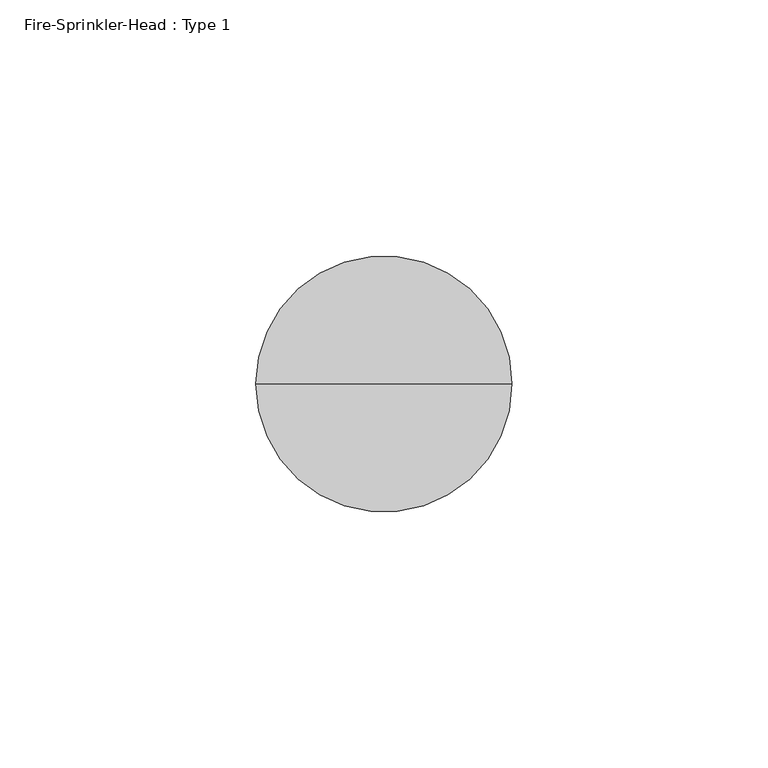
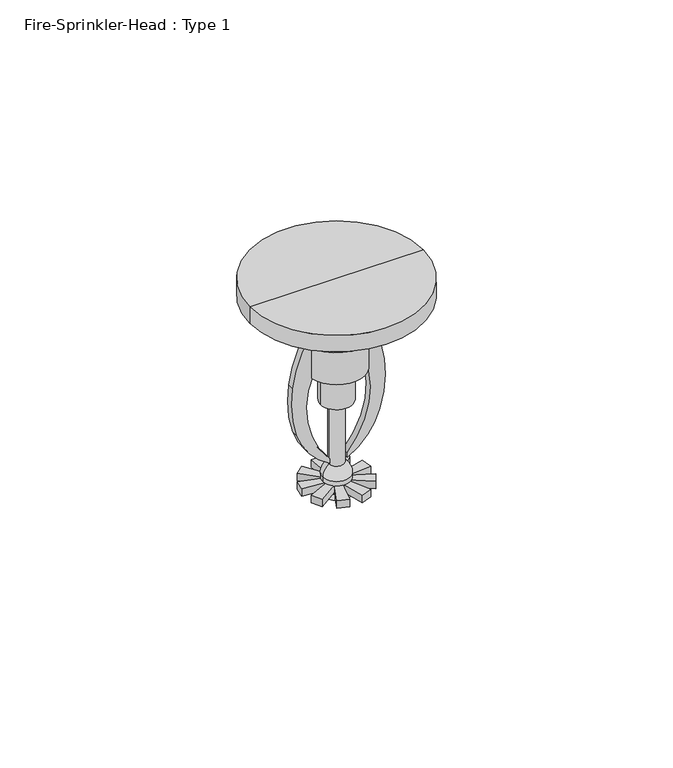
"""IFC4 building model written with IfcOpenShell, lengths in millimetres: alarm geometry, Fire-Sprinkler-Head : Type 1."""

import ifcopenshell
import ifcopenshell.guid

model = None  # the IFC model being written
_history = None  # IfcOwnerHistory: only IFC2X3 demands one
_inside = {}  # id of a spatial element -> (the spatial element, [elements in it])
_under = {}  # id of a project, library or spatial element -> (it, [spatial elements below it])
_declared = {}  # id of a project -> (the project, [libraries it declares])
_typed = {}  # id of a type object -> (the type object, [elements of that type])
_made_of = {}  # id of a material, layer set ... -> (it, [elements and type objects made of it])


def new_model(schema):
    """Start an empty IFC model of exactly this schema.

    Asked for "IFC4X3", IfcOpenShell would pick the latest addendum, in which some entities
    have other attributes; the version numbers below select the first issue.
    IFC2X3 requires an IfcOwnerHistory on every rooted entity: one is made here for all.
    """
    global model, _history
    if schema == "IFC4X3":
        model = ifcopenshell.file(schema_version=(4, 3, 0, 0))
    else:
        model = ifcopenshell.file(schema=schema)
    _inside.clear()
    _under.clear()
    _declared.clear()
    _typed.clear()
    _made_of.clear()
    _history = None
    if model.schema == "IFC2X3":
        org = make("IfcOrganization", Name="unknown")
        user = make(
            "IfcPersonAndOrganization",
            ThePerson=make("IfcPerson", FamilyName="unknown"),
            TheOrganization=org,
        )
        app = make(
            "IfcApplication",
            ApplicationDeveloper=org,
            Version="unknown",
            ApplicationFullName="unknown",
            ApplicationIdentifier="unknown",
        )
        _history = make(
            "IfcOwnerHistory",
            OwningUser=user,
            OwningApplication=app,
            ChangeAction="ADDED",
            CreationDate=0,
        )
    return model


def make(cls, **values):
    """One entity of the class cls with the attributes given. An attribute that is None is left unset."""
    return model.create_entity(
        cls, **{name: value for name, value in values.items() if value is not None}
    )


def rooted(cls, **values):
    """An entity with a GlobalId (a new one), such as an element, a storey or a relation."""
    return make(cls, GlobalId=ifcopenshell.guid.new(), OwnerHistory=_history, **values)


def si_unit(unit_type, name, prefix=None):
    """IfcSIUnit, for example si_unit("LENGTHUNIT", "METRE", prefix="MILLI")."""
    return make("IfcSIUnit", UnitType=unit_type, Prefix=prefix, Name=name)


def assignment(units):
    """IfcUnitAssignment: the units of a project."""
    return None if units is None else make("IfcUnitAssignment", Units=units)


def point(xyz):
    """IfcCartesianPoint."""
    return None if xyz is None else make("IfcCartesianPoint", Coordinates=xyz)


def direction(xyz):
    """IfcDirection."""
    return None if xyz is None else make("IfcDirection", DirectionRatios=xyz)


def frame(location, z_axis=None, x_axis=None):
    """IfcAxis2Placement3D, a coordinate frame: its origin and axes. An axis left out is left unset."""
    return make(
        "IfcAxis2Placement3D",
        Location=point(location),
        Axis=direction(z_axis),
        RefDirection=direction(x_axis),
    )


def frame_2d(location, x_axis=None):
    """IfcAxis2Placement2D, a coordinate frame in the plane: its origin and x axis."""
    return make(
        "IfcAxis2Placement2D", Location=point(location), RefDirection=direction(x_axis)
    )


def origin():
    """The frame at (0, 0, 0) with its axes left unset."""
    return frame((0.0, 0.0, 0.0))


def place(relative_to, where):
    """IfcLocalPlacement: puts the frame where relative to a parent placement (None: the world)."""
    return make(
        "IfcLocalPlacement", PlacementRelTo=relative_to, RelativePlacement=where
    )


def context(
    kind, dimensions, precision=None, world=None, true_north=None, identifier=None
):
    """IfcGeometricRepresentationContext, for example the 3D "Model" context."""
    return make(
        "IfcGeometricRepresentationContext",
        ContextIdentifier=identifier,
        ContextType=kind,
        CoordinateSpaceDimension=dimensions,
        Precision=precision,
        WorldCoordinateSystem=world,
        TrueNorth=true_north,
    )


def project(units=None, contexts=None):
    """IfcProject with its units and contexts."""
    return rooted(
        "IfcProject",
        Name="project",
        RepresentationContexts=contexts,
        UnitsInContext=assignment(units),
    )


def spatial(cls, under=None, at=None, **own):
    """A site, building, storey or space (cls), placed at a placement, below another one or the project."""
    s = rooted(cls, ObjectPlacement=at, **own)
    if under is not None:
        _under.setdefault(under.id(), (under, []))[1].append(s)
    return s


def polyline(points):
    """IfcPolyline through the points."""
    return make("IfcPolyline", Points=[point(p) for p in points])


def circle_curve(where, radius):
    """IfcCircle in the frame where."""
    return make("IfcCircle", Position=where, Radius=radius)


def ellipse_curve(where, semi_axis1, semi_axis2):
    """IfcEllipse in the frame where."""
    return make(
        "IfcEllipse", Position=where, SemiAxis1=semi_axis1, SemiAxis2=semi_axis2
    )


def trimmed(basis, trim1, trim2, sense, master):
    """IfcTrimmedCurve: the piece of a basis curve between two trims."""
    return make(
        "IfcTrimmedCurve",
        BasisCurve=basis,
        Trim1=trim1,
        Trim2=trim2,
        SenseAgreement=sense,
        MasterRepresentation=master,
    )


def segment(curve, same_sense, transition):
    """IfcCompositeCurveSegment."""
    return make(
        "IfcCompositeCurveSegment",
        Transition=transition,
        SameSense=same_sense,
        ParentCurve=curve,
    )


def composite_curve(segments, self_intersect=None):
    """IfcCompositeCurve: segments joined end to end."""
    return make("IfcCompositeCurve", Segments=segments, SelfIntersect=self_intersect)


def outline(outer, holes=None, kind="AREA"):
    """IfcArbitraryClosedProfileDef: a profile drawn as a closed curve; with holes, ...WithVoids."""
    if holes is None:
        return make("IfcArbitraryClosedProfileDef", ProfileType=kind, OuterCurve=outer)
    return make(
        "IfcArbitraryProfileDefWithVoids",
        ProfileType=kind,
        OuterCurve=outer,
        InnerCurves=holes,
    )


def extrude(swept, where, along, depth):
    """IfcExtrudedAreaSolid: the profile swept, set in the frame where, extruded along a direction by depth."""
    return make(
        "IfcExtrudedAreaSolid",
        SweptArea=swept,
        Position=where,
        ExtrudedDirection=direction(along),
        Depth=depth,
    )


def shape(context_of_items, identifier, shape_type, items):
    """IfcShapeRepresentation: the items that make up one representation, for example the "Body"."""
    return make(
        "IfcShapeRepresentation",
        ContextOfItems=context_of_items,
        RepresentationIdentifier=identifier,
        RepresentationType=shape_type,
        Items=items,
    )


def source(mapping_origin, context_of_items, identifier, shape_type, items):
    """IfcRepresentationMap: a shape defined once, which mapped items show again and again."""
    return make(
        "IfcRepresentationMap",
        MappingOrigin=mapping_origin,
        MappedRepresentation=shape(context_of_items, identifier, shape_type, items),
    )


def transform(
    local_origin,
    x_axis=None,
    y_axis=None,
    z_axis=None,
    scale=None,
    scale2=None,
    scale3=None,
    uniform=True,
):
    """IfcCartesianTransformationOperator3D, or its non-uniform kind. x_axis, y_axis, z_axis: its Axis1, 2, 3."""
    if uniform:
        return make(
            "IfcCartesianTransformationOperator3D",
            Axis1=direction(x_axis),
            Axis2=direction(y_axis),
            LocalOrigin=point(local_origin),
            Scale=scale,
            Axis3=direction(z_axis),
        )
    return make(
        "IfcCartesianTransformationOperator3DnonUniform",
        Axis1=direction(x_axis),
        Axis2=direction(y_axis),
        LocalOrigin=point(local_origin),
        Scale=scale,
        Axis3=direction(z_axis),
        Scale2=scale2,
        Scale3=scale3,
    )


def mapped(mapping_source, mapping_target):
    """IfcMappedItem: shows the shape of a source again, moved by a transform."""
    return make(
        "IfcMappedItem", MappingSource=mapping_source, MappingTarget=mapping_target
    )


def made_of(thing, what):
    """Note that an element or type object is made of a material, layer set ...; save() writes the relation."""
    if what is not None:
        _made_of.setdefault(what.id(), (what, []))[1].append(thing)
    return thing


def element(
    cls,
    number,
    at=None,
    inside=None,
    cuts=None,
    type_object=None,
    material=None,
    context=None,
    identifier="Body",
    shape_type=None,
    held_by="IfcProductDefinitionShape",
    body=None,
    shapes=None,
    **own,
):
    """One element of the class cls, such as IfcWall. Its Tag is "e" and its number.

    at: its placement. inside: the storey or other place that contains it. cuts: it is an
    opening in that element (IfcRelVoidsElement). A single representation is given by context,
    identifier, shape_type and body (its items); several are given by shapes. held_by: the class
    of the entity that holds the representations. save() writes the other relations.
    """
    e = rooted(cls, Tag="e%d" % number, ObjectPlacement=at, **own)
    if body is not None:
        shapes = [shape(context, identifier, shape_type, body)]
    if shapes is not None:
        e.Representation = make(held_by, Representations=shapes)
    if inside is not None:
        _inside.setdefault(inside.id(), (inside, []))[1].append(e)
    if cuts is not None:
        rooted(
            "IfcRelVoidsElement", RelatingBuildingElement=cuts, RelatedOpeningElement=e
        )
    if type_object is not None:
        _typed.setdefault(type_object.id(), (type_object, []))[1].append(e)
    return made_of(e, material)


def aggregate(whole, parts):
    """IfcRelAggregates: a whole, such as a stair, and the parts it consists of."""
    return rooted("IfcRelAggregates", RelatingObject=whole, RelatedObjects=parts)


def save(model, path):
    """Write the relations noted so far, then the file.

    IfcRelAggregates (storeys below a building ...), IfcRelContainedInSpatialStructure (elements
    in a storey), IfcRelDefinesByType, IfcRelAssociatesMaterial and IfcRelDeclares: one each for
    every whole, place, type object, material and project.
    """
    for whole, parts in _under.values():
        aggregate(whole, parts)
    for where, things in _inside.values():
        rooted(
            "IfcRelContainedInSpatialStructure",
            RelatedElements=things,
            RelatingStructure=where,
        )
    for kind, things in _typed.values():
        rooted("IfcRelDefinesByType", RelatedObjects=things, RelatingType=kind)
    for what, things in _made_of.values():
        rooted("IfcRelAssociatesMaterial", RelatedObjects=things, RelatingMaterial=what)
    for by, libraries in _declared.values():
        rooted("IfcRelDeclares", RelatingContext=by, RelatedDefinitions=libraries)
    model.write(path)


def plane_surface(at):
    """IfcPlane: the flat surface through the origin of the frame at, square to its z axis."""
    return make("IfcPlane", Position=at)


def cylinder_surface(at, radius):
    """IfcCylindricalSurface: all points at the distance radius from the z axis of the frame at."""
    return make("IfcCylindricalSurface", Position=at, Radius=radius)


def revolved_surface(curve, axis_point, axis_direction):
    """IfcSurfaceOfRevolution: the curve turned about the line through axis_point along axis_direction."""
    return make(
        "IfcSurfaceOfRevolution",
        SweptCurve=make("IfcArbitraryOpenProfileDef", ProfileType="CURVE", Curve=curve),
        AxisPosition=make("IfcAxis1Placement", Location=point(axis_point), Axis=direction(axis_direction)),
    )


def advanced_brep(points, edges, surfaces, faces):
    """IfcAdvancedBrep: a solid bounded by faces that lie on surfaces and meet in shared edges.

    An edge is (start, end): straight between two places in points (the first is 0);
    or (start, end, curve); or (start, end, curve, False) where it runs against its curve.
    A face is (place in surfaces, loops), or (place, loops, False) where it looks against
    its surface's normal. A loop lists edges by number (the first is 1), with a minus sign
    where the edge is run from its end to its start. The first loop is the outer one.
    """
    corners = [point(p) for p in points]
    vertices = [make("IfcVertexPoint", VertexGeometry=c) for c in corners]
    made = []
    for start, end, *more in edges:
        made.append(
            make(
                "IfcEdgeCurve",
                EdgeStart=vertices[start],
                EdgeEnd=vertices[end],
                EdgeGeometry=more[0] if more else make("IfcPolyline", Points=[corners[start], corners[end]]),
                SameSense=more[1] if len(more) > 1 else True,
            )
        )
    hull = []
    for where, loops, *sense in faces:
        bounds = []
        for j, loop in enumerate(loops):
            ring = [make("IfcOrientedEdge", EdgeElement=made[abs(k) - 1], Orientation=k > 0) for k in loop]
            bounds.append(
                make(
                    "IfcFaceOuterBound" if j == 0 else "IfcFaceBound",
                    Bound=make("IfcEdgeLoop", EdgeList=ring),
                    Orientation=True,
                )
            )
        hull.append(make("IfcAdvancedFace", Bounds=bounds, FaceSurface=surfaces[where], SameSense=sense[0] if sense else True))
    return make("IfcAdvancedBrep", Outer=make("IfcClosedShell", CfsFaces=hull))


def fire_sprinkler_head_type_1_89d12226(model_context):
    return source(origin(), model_context, "Body", "SolidModel", [
        extrude(outline(composite_curve([segment(polyline([(3978.349287, 0.0), (3978.349287, 4.8492465)]), True, "CONTINUOUS"), segment(trimmed(circle_curve(frame_2d((3963.8626562, -16.7101966)), 25.9744501), [point((3978.349287, 4.8492465))], [point((3946.4410747, 2.555331))], True, "CARTESIAN"), True, "CONTINUOUS"), segment(polyline([(3946.4410747, 2.555331), (3945.0501011, 2.555331)]), True, "CONTINUOUS"), segment(trimmed(circle_curve(frame_2d((3962.5874819, -7.1839127)), 20.0602242), [point((3945.0501011, 2.555331))], [point((3956.7072905, 11.9951369))], False, "CARTESIAN"), True, "CONTINUOUS"), segment(trimmed(circle_curve(frame_2d((3966.9398015, -21.3795994)), 34.9081266), [point((3956.7072905, 11.9951369))], [point((3971.4511948, 13.2357821))], False, "CARTESIAN"), True, "CONTINUOUS"), segment(trimmed(circle_curve(frame_2d((3966.6562283, -22.8835825)), 36.4362484), [point((3971.4511948, 13.2357821))], [point((3985.8319856, 8.0985177))], False, "CARTESIAN"), True, "CONTINUOUS"), segment(polyline([(3985.8319856, 8.0985177), (3985.8319856, 0.0), (3978.349287, 0.0)]), True, "CONTINUOUS")], self_intersect=False)), frame((0.0, -0.987392, 0.0), z_axis=(0.0, 1.0, 0.0), x_axis=(0.0, 0.0, 1.0)), (0.0, 0.0, 1.0), 2.0345161),
        extrude(outline(polyline([(9.9808686, 0.1084998), (0.132791, -0.7530953), (-0.132791, 0.7530953), (9.4160577, 3.3117016), (9.9808686, 0.1084998)])), frame((0.0, 0.0, 3936.8211831), z_axis=(0.0, 0.0, 1.0), x_axis=(1.0, 0.0, 0.0)), (0.0, 0.0, 1.0), 2.2906652),
        extrude(outline(polyline([(7.7155312, -6.332463), (-0.3823565, -0.6622609), (0.3823565, 0.6622609), (9.3418394, -3.5156146), (7.7155312, -6.332463)])), frame((0.0, 0.0, 3936.8211831), z_axis=(0.0, 0.0, 1.0), x_axis=(1.0, 0.0, 0.0)), (0.0, 0.0, 1.0), 2.2906652),
        extrude(outline(polyline([(1.8400111, -9.8103959), (-0.7185952, -0.2615473), (0.7185952, 0.2615473), (4.8964707, -8.6979356), (1.8400111, -9.8103959)])), frame((0.0, 0.0, 3936.8211831), z_axis=(0.0, 0.0, 1.0), x_axis=(1.0, 0.0, 0.0)), (0.0, 0.0, 1.0), 2.2906652),
        extrude(outline(polyline([(-4.8964707, -8.6979356), (-0.7185952, 0.2615473), (0.7185952, -0.2615473), (-1.8400111, -9.8103959), (-4.8964707, -8.6979356)])), frame((0.0, 0.0, 3936.8211831), z_axis=(0.0, 0.0, 1.0), x_axis=(1.0, 0.0, 0.0)), (0.0, 0.0, 1.0), 2.2906652),
        extrude(outline(polyline([(-9.3418394, -3.5156146), (-0.3823565, 0.6622609), (0.3823565, -0.6622609), (-7.7155312, -6.332463), (-9.3418394, -3.5156146)])), frame((0.0, 0.0, 3936.8211831), z_axis=(0.0, 0.0, 1.0), x_axis=(1.0, 0.0, 0.0)), (0.0, 0.0, 1.0), 2.2906652),
        extrude(outline(polyline([(-9.4160577, 3.3117016), (0.132791, 0.7530953), (-0.132791, -0.7530953), (-9.9808686, 0.1084998), (-9.4160577, 3.3117016)])), frame((0.0, 0.0, 3936.8211831), z_axis=(0.0, 0.0, 1.0), x_axis=(1.0, 0.0, 0.0)), (0.0, 0.0, 1.0), 2.2906652),
        extrude(outline(polyline([(-5.0843979, 8.5894358), (0.5858042, 0.4915481), (-0.5858042, -0.4915481), (-7.5760466, 6.4986943), (-5.0843979, 8.5894358)])), frame((0.0, 0.0, 3936.8211831), z_axis=(0.0, 0.0, 1.0), x_axis=(1.0, 0.0, 0.0)), (0.0, 0.0, 1.0), 2.2906652),
        extrude(outline(polyline([(7.5760466, 6.4986943), (0.5858042, -0.4915481), (-0.5858042, 0.4915481), (5.0843979, 8.5894358), (7.5760466, 6.4986943)])), frame((0.0, 0.0, 3936.8211831), z_axis=(0.0, 0.0, 1.0), x_axis=(1.0, 0.0, 0.0)), (0.0, 0.0, 1.0), 2.2906652),
        extrude(outline(polyline([(1.6263082, 9.8480775), (0.764713, 0.0), (-0.764713, 0.0), (-1.6263082, 9.8480775), (1.6263082, 9.8480775)])), frame((0.0, 0.0, 3936.8211831), z_axis=(0.0, 0.0, 1.0), x_axis=(1.0, 0.0, 0.0)), (0.0, 0.0, 1.0), 2.2906652),
        extrude(outline(composite_curve([segment(polyline([(3978.349287, 0.0), (3985.8319856, 0.0), (3985.8319856, -8.0985177)]), True, "CONTINUOUS"), segment(trimmed(circle_curve(frame_2d((3966.6562283, 22.8835825)), 36.4362484), [point((3985.8319856, -8.0985177))], [point((3971.4511948, -13.2357821))], False, "CARTESIAN"), True, "CONTINUOUS"), segment(trimmed(circle_curve(frame_2d((3966.9398015, 21.3795994)), 34.9081266), [point((3971.4511948, -13.2357821))], [point((3956.7072905, -11.9951369))], False, "CARTESIAN"), True, "CONTINUOUS"), segment(trimmed(circle_curve(frame_2d((3962.5874819, 7.1839127)), 20.0602242), [point((3956.7072905, -11.9951369))], [point((3945.0501011, -2.555331))], False, "CARTESIAN"), True, "CONTINUOUS"), segment(polyline([(3945.0501011, -2.555331), (3946.4410747, -2.555331)]), True, "CONTINUOUS"), segment(trimmed(circle_curve(frame_2d((3963.8626562, 16.7101966)), 25.9744501), [point((3946.4410747, -2.555331))], [point((3978.349287, -4.8492465))], True, "CARTESIAN"), True, "CONTINUOUS"), segment(polyline([(3978.349287, -4.8492465), (3978.349287, 0.0)]), True, "CONTINUOUS")], self_intersect=False)), frame((0.0, -0.987392, 0.0), z_axis=(0.0, 1.0, 0.0), x_axis=(0.0, 0.0, 1.0)), (0.0, 0.0, 1.0), 2.0345161),
        advanced_brep(
        [(25.0, 0.0, 3995.0), (-25.0, 0.0, 3995.0), (-25.0, 0.0, 4000.0), (25.0, 0.0, 4000.0), (18.8042198, 0.0, 3995.0), (-18.8042198, 0.0, 3995.0), (12.2416631, 0.0, 3991.6324601), (-12.2416631, 0.0, 3991.6324601), (12.2416631, 0.0, 3985.8319856), (-12.2416631, 0.0, 3985.8319856), (8.0985177, 0.0, 3985.8319856), (-8.0985177, 0.0, 3985.8319856), (8.0985177, 0.0, 3973.1223694), (-8.0985177, 0.0, 3973.1223694), (4.6513455, 0.0, 3973.1223694), (-4.6513455, 0.0, 3973.1223694), (4.6513455, 0.0, 3963.1223694), (-4.6513455, 0.0, 3963.1223694), (2.1931757, 0.0, 3963.1223694), (-2.1931757, 0.0, 3963.1223694), (2.1931757, 0.0, 3944.1533344), (-2.1931757, 0.0, 3944.1533344), (4.0228103, 0.0, 3940.7527841), (-4.0228103, 0.0, 3940.7527841), (4.0228103, 0.0, 3939.1118483), (-4.0228103, 0.0, 3939.1118483), (1.2979197, 0.0, 3939.1118483), (-1.2979197, 0.0, 3939.1118483), (1.2979197, 0.0, 3936.9618068), (-1.2979197, 0.0, 3936.9618068), (4.3349972, 0.0, 3936.9618068), (-4.3349972, 0.0, 3936.9618068), (4.3349972, 0.0, 3935.4284458), (-4.3349972, 0.0, 3935.4284458), (0.0, 0.0, 3935.4284458), (0.0, 0.0, 4000.0)],
        [
            (0, 1, circle_curve(frame((0.0, 0.0, 3995.0), z_axis=(0.0, 0.0, 1.0), x_axis=(-1.0, 0.0, 0.0)), 25.0)),
            (1, 2),
            (2, 3, circle_curve(frame((0.0, 0.0, 4000.0), z_axis=(0.0, 0.0, -1.0), x_axis=(-1.0, 0.0, 0.0)), 25.0)),
            (3, 0),
            (1, 0, circle_curve(frame((0.0, 0.0, 3995.0), z_axis=(0.0, 0.0, 1.0), x_axis=(-1.0, 0.0, 0.0)), 25.0)),
            (3, 2, circle_curve(frame((0.0, 0.0, 4000.0), z_axis=(0.0, 0.0, -1.0), x_axis=(-1.0, 0.0, 0.0)), 25.0)),
            (4, 5, circle_curve(frame((0.0, 0.0, 3995.0), z_axis=(0.0, 0.0, 1.0), x_axis=(-1.0, 0.0, 0.0)), 18.8042198)),
            (5, 1),
            (0, 4),
            (5, 4, circle_curve(frame((0.0, 0.0, 3995.0), z_axis=(0.0, 0.0, 1.0), x_axis=(-1.0, 0.0, 0.0)), 18.8042198)),
            (6, 7, circle_curve(frame((0.0, 0.0, 3991.6324601), z_axis=(0.0, 0.0, 1.0), x_axis=(-1.0, 0.0, 0.0)), 12.2416631)),
            (7, 5, circle_curve(frame((-4.8124083, 0.0, 4014.1885825), z_axis=(0.0, 1.0, 0.0), x_axis=(-1.0, 0.0, 0.0)), 23.7481049)),
            (4, 6, circle_curve(frame((4.8124083, 0.0, 4014.1885825), z_axis=(0.0, 1.0, 0.0), x_axis=(1.0, 0.0, 0.0)), 23.7481049)),
            (7, 6, circle_curve(frame((0.0, 0.0, 3991.6324601), z_axis=(0.0, 0.0, 1.0), x_axis=(-1.0, 0.0, 0.0)), 12.2416631)),
            (8, 9, circle_curve(frame((0.0, 0.0, 3985.8319856), z_axis=(0.0, 0.0, 1.0), x_axis=(-1.0, 0.0, 0.0)), 12.2416631)),
            (9, 7),
            (6, 8),
            (9, 8, circle_curve(frame((0.0, 0.0, 3985.8319856), z_axis=(0.0, 0.0, 1.0), x_axis=(-1.0, 0.0, 0.0)), 12.2416631)),
            (10, 11, circle_curve(frame((0.0, 0.0, 3985.8319856), z_axis=(0.0, 0.0, 1.0), x_axis=(-1.0, 0.0, 0.0)), 8.0985177)),
            (11, 9),
            (8, 10),
            (11, 10, circle_curve(frame((0.0, 0.0, 3985.8319856), z_axis=(0.0, 0.0, 1.0), x_axis=(-1.0, 0.0, 0.0)), 8.0985177)),
            (12, 13, circle_curve(frame((0.0, 0.0, 3973.1223694), z_axis=(0.0, 0.0, 1.0), x_axis=(-1.0, 0.0, 0.0)), 8.0985177)),
            (13, 11),
            (10, 12),
            (13, 12, circle_curve(frame((0.0, 0.0, 3973.1223694), z_axis=(0.0, 0.0, 1.0), x_axis=(-1.0, 0.0, 0.0)), 8.0985177)),
            (14, 15, circle_curve(frame((0.0, 0.0, 3973.1223694), z_axis=(0.0, 0.0, 1.0), x_axis=(-1.0, 0.0, 0.0)), 4.6513455)),
            (15, 13),
            (12, 14),
            (15, 14, circle_curve(frame((0.0, 0.0, 3973.1223694), z_axis=(0.0, 0.0, 1.0), x_axis=(-1.0, 0.0, 0.0)), 4.6513455)),
            (16, 17, circle_curve(frame((0.0, 0.0, 3963.1223694), z_axis=(0.0, 0.0, 1.0), x_axis=(-1.0, 0.0, 0.0)), 4.6513455)),
            (17, 15),
            (14, 16),
            (17, 16, circle_curve(frame((0.0, 0.0, 3963.1223694), z_axis=(0.0, 0.0, 1.0), x_axis=(-1.0, 0.0, 0.0)), 4.6513455)),
            (18, 19, circle_curve(frame((0.0, 0.0, 3963.1223694), z_axis=(0.0, 0.0, 1.0), x_axis=(-1.0, 0.0, 0.0)), 2.1931757)),
            (19, 17),
            (16, 18),
            (19, 18, circle_curve(frame((0.0, 0.0, 3963.1223694), z_axis=(0.0, 0.0, 1.0), x_axis=(-1.0, 0.0, 0.0)), 2.1931757)),
            (20, 21, circle_curve(frame((0.0, 0.0, 3944.1533344), z_axis=(0.0, 0.0, 1.0), x_axis=(-1.0, 0.0, 0.0)), 2.1931757)),
            (21, 19),
            (18, 20),
            (21, 20, circle_curve(frame((0.0, 0.0, 3944.1533344), z_axis=(0.0, 0.0, 1.0), x_axis=(-1.0, 0.0, 0.0)), 2.1931757)),
            (22, 23, circle_curve(frame((0.0, 0.0, 3940.7527841), z_axis=(0.0, 0.0, 1.0), x_axis=(-1.0, 0.0, 0.0)), 4.0228103)),
            (23, 21, circle_curve(frame((0.3386488, 0.0, 3940.5986256), z_axis=(0.0, 1.0, 0.0), x_axis=(-1.0, 0.0, 0.0)), 4.3641826)),
            (20, 22, circle_curve(frame((-0.3386488, 0.0, 3940.5986256), z_axis=(0.0, 1.0, 0.0), x_axis=(1.0, 0.0, 0.0)), 4.3641826)),
            (23, 22, circle_curve(frame((0.0, 0.0, 3940.7527841), z_axis=(0.0, 0.0, 1.0), x_axis=(-1.0, 0.0, 0.0)), 4.0228103)),
            (24, 25, circle_curve(frame((0.0, 0.0, 3939.1118483), z_axis=(0.0, 0.0, 1.0), x_axis=(-1.0, 0.0, 0.0)), 4.0228103)),
            (25, 23),
            (22, 24),
            (25, 24, circle_curve(frame((0.0, 0.0, 3939.1118483), z_axis=(0.0, 0.0, 1.0), x_axis=(-1.0, 0.0, 0.0)), 4.0228103)),
            (26, 27, circle_curve(frame((0.0, 0.0, 3939.1118483), z_axis=(0.0, 0.0, 1.0), x_axis=(-1.0, 0.0, 0.0)), 1.2979197)),
            (27, 25),
            (24, 26),
            (27, 26, circle_curve(frame((0.0, 0.0, 3939.1118483), z_axis=(0.0, 0.0, 1.0), x_axis=(-1.0, 0.0, 0.0)), 1.2979197)),
            (28, 29, circle_curve(frame((0.0, 0.0, 3936.9618068), z_axis=(0.0, 0.0, 1.0), x_axis=(-1.0, 0.0, 0.0)), 1.2979197)),
            (29, 27),
            (26, 28),
            (29, 28, circle_curve(frame((0.0, 0.0, 3936.9618068), z_axis=(0.0, 0.0, 1.0), x_axis=(-1.0, 0.0, 0.0)), 1.2979197)),
            (30, 31, circle_curve(frame((0.0, 0.0, 3936.9618068), z_axis=(0.0, 0.0, 1.0), x_axis=(-1.0, 0.0, 0.0)), 4.3349972)),
            (31, 29),
            (28, 30),
            (31, 30, circle_curve(frame((0.0, 0.0, 3936.9618068), z_axis=(0.0, 0.0, 1.0), x_axis=(-1.0, 0.0, 0.0)), 4.3349972)),
            (32, 33, circle_curve(frame((0.0, 0.0, 3935.4284458), z_axis=(0.0, 0.0, 1.0), x_axis=(-1.0, 0.0, 0.0)), 4.3349972)),
            (33, 31, circle_curve(frame((-4.3349972, 0.0, 3936.1951263), z_axis=(0.0, 1.0, 0.0), x_axis=(-1.0, 0.0, 0.0)), 0.7666805)),
            (30, 32, circle_curve(frame((4.3349972, 0.0, 3936.1951263), z_axis=(0.0, 1.0, 0.0), x_axis=(1.0, 0.0, 0.0)), 0.7666805)),
            (33, 32, circle_curve(frame((0.0, 0.0, 3935.4284458), z_axis=(0.0, 0.0, 1.0), x_axis=(-1.0, 0.0, 0.0)), 4.3349972)),
            (34, 33),
            (32, 34),
            (2, 35),
            (35, 3),
        ],
        [
            cylinder_surface(frame((0.0, 0.0, 3925.1994284), z_axis=(0.0, 0.0, -1.0), x_axis=(-1.0, 0.0, 0.0)), 25.0),
            plane_surface(frame((0.0, 0.0, 3995.0), z_axis=(0.0, 0.0, -1.0), x_axis=(-1.0, 0.0, 0.0))),
            revolved_surface(trimmed(ellipse_curve(frame((-4.8124083, 0.0, 4014.1885825), z_axis=(0.0, -1.0, 0.0), x_axis=(-1.0, 0.0, 0.0)), 23.7481049, 23.7481049), [point((-18.8042198, 0.0, 3995.0))], [point((-12.2416631, 0.0, 3991.6324601))], True, "CARTESIAN"), (0.0, 0.0, 3925.1994284), (0.0, 0.0, -1.0)),
            cylinder_surface(frame((0.0, 0.0, 3925.1994284), z_axis=(0.0, 0.0, -1.0), x_axis=(-1.0, 0.0, 0.0)), 12.2416631),
            plane_surface(frame((0.0, 0.0, 3985.8319856), z_axis=(0.0, 0.0, -1.0), x_axis=(-1.0, 0.0, 0.0))),
            cylinder_surface(frame((0.0, 0.0, 3925.1994284), z_axis=(0.0, 0.0, -1.0), x_axis=(-1.0, 0.0, 0.0)), 8.0985177),
            plane_surface(frame((0.0, 0.0, 3973.1223694), z_axis=(0.0, 0.0, -1.0), x_axis=(-1.0, 0.0, 0.0))),
            cylinder_surface(frame((0.0, 0.0, 3925.1994284), z_axis=(0.0, 0.0, -1.0), x_axis=(-1.0, 0.0, 0.0)), 4.6513455),
            plane_surface(frame((0.0, 0.0, 3963.1223694), z_axis=(0.0, 0.0, -1.0), x_axis=(-1.0, 0.0, 0.0))),
            cylinder_surface(frame((0.0, 0.0, 3925.1994284), z_axis=(0.0, 0.0, -1.0), x_axis=(-1.0, 0.0, 0.0)), 2.1931757),
            revolved_surface(trimmed(ellipse_curve(frame((0.3386488, 0.0, 3940.5986256), z_axis=(0.0, -1.0, 0.0), x_axis=(-1.0, 0.0, 0.0)), 4.3641826, 4.3641826), [point((-2.1931757, 0.0, 3944.1533344))], [point((-4.0228103, 0.0, 3940.7527841))], True, "CARTESIAN"), (0.0, 0.0, 3925.1994284), (0.0, 0.0, -1.0)),
            cylinder_surface(frame((0.0, 0.0, 3925.1994284), z_axis=(0.0, 0.0, -1.0), x_axis=(-1.0, 0.0, 0.0)), 4.0228103),
            plane_surface(frame((0.0, 0.0, 3939.1118483), z_axis=(0.0, 0.0, -1.0), x_axis=(-1.0, 0.0, 0.0))),
            cylinder_surface(frame((0.0, 0.0, 3925.1994284), z_axis=(0.0, 0.0, -1.0), x_axis=(-1.0, 0.0, 0.0)), 1.2979197),
            plane_surface(frame((0.0, 0.0, 3936.9618068), z_axis=(0.0, 0.0, 1.0), x_axis=(-1.0, 0.0, 0.0))),
            revolved_surface(trimmed(ellipse_curve(frame((-4.3349972, 0.0, 3936.1951263), z_axis=(0.0, -1.0, 0.0), x_axis=(-1.0, 0.0, 0.0)), 0.7666805, 0.7666805), [point((-4.3349972, 0.0, 3936.9618068))], [point((-4.3349972, 0.0, 3935.4284458))], True, "CARTESIAN"), (0.0, 0.0, 3925.1994284), (0.0, 0.0, -1.0)),
            plane_surface(frame((0.0, 0.0, 3935.4284458), z_axis=(0.0, 0.0, -1.0), x_axis=(-1.0, 0.0, 0.0))),
            plane_surface(frame((0.0, 0.0, 4000.0), z_axis=(0.0, 0.0, 1.0), x_axis=(-1.0, 0.0, 0.0))),
        ],
        [
            (0, [[1, 2, 3, 4]]),
            (0, [[5, -4, 6, -2]]),
            (1, [[7, 8, -1, 9]]),
            (1, [[10, -9, -5, -8]]),
            (2, [[11, 12, -7, 13]]),
            (2, [[14, -13, -10, -12]]),
            (3, [[15, 16, -11, 17]]),
            (3, [[18, -17, -14, -16]]),
            (4, [[19, 20, -15, 21]]),
            (4, [[22, -21, -18, -20]]),
            (5, [[23, 24, -19, 25]]),
            (5, [[26, -25, -22, -24]]),
            (6, [[27, 28, -23, 29]]),
            (6, [[30, -29, -26, -28]]),
            (7, [[31, 32, -27, 33]]),
            (7, [[34, -33, -30, -32]]),
            (8, [[35, 36, -31, 37]]),
            (8, [[38, -37, -34, -36]]),
            (9, [[39, 40, -35, 41]]),
            (9, [[42, -41, -38, -40]]),
            (10, [[43, 44, -39, 45]]),
            (10, [[46, -45, -42, -44]]),
            (11, [[47, 48, -43, 49]]),
            (11, [[50, -49, -46, -48]]),
            (12, [[51, 52, -47, 53]]),
            (12, [[54, -53, -50, -52]]),
            (13, [[55, 56, -51, 57]]),
            (13, [[58, -57, -54, -56]]),
            (14, [[59, 60, -55, 61]]),
            (14, [[62, -61, -58, -60]]),
            (15, [[63, 64, -59, 65]]),
            (15, [[66, -65, -62, -64]]),
            (16, [[67, -63, 68]]),
            (16, [[-68, -66, -67]]),
            (17, [[-3, 69, 70]]),
            (17, [[-6, -70, -69]]),
        ],
    ),
    ])


if __name__ == "__main__":
    model = new_model("IFC4")
    model_context = context("Model", 3, world=origin())
    ifc_project = project(units=[si_unit("LENGTHUNIT", "METRE", prefix="MILLI")], contexts=[model_context])
    site = spatial("IfcSite", under=ifc_project)
    building = spatial("IfcBuilding", under=site)
    placement = place(None, origin())
    fire_sprinkler_head_type_1_shape = fire_sprinkler_head_type_1_89d12226(model_context)
    element("IfcAlarm", 1, ObjectType="Fire-Sprinkler-Head : Type 1", at=placement, inside=building, context=model_context, shape_type="MappedRepresentation", body=[
        mapped(fire_sprinkler_head_type_1_shape, transform((0.0, 0.0, 0.0), x_axis=(1.0, 0.0, 0.0), y_axis=(0.0, 1.0, 0.0), z_axis=(0.0, 0.0, 1.0))),
    ])
    save(model, "model.ifc")

# Revit data of these elements
# Type "Fire-Sprinkler-Head : Type 1"
#   URL = "http://www.arcat.com/"
#   Test Data = ""
#   Temp Range = "50F / 100F over Ambient"
#   Specification = "http://www.arcat.com/divs/sec/sec13930.shtml"
#   Sales Information = ""
#   Product Properties = "http://www.arcat.com/bim/bim_info.pl?fn=Fire-Sprinkler-Head"
#   Product Data = "http://www.arcat.com/divs/sec/sec13930.shtml"
#   Model = "Generic"
#   Manufacturer Website = "http://www.arcat.com/"
#   Manufacturer Phone - Toll Free = ""
#   Manufacturer Phone = "(203) 929-9444"
#   Manufacturer Fax = "(203) 929-9444"
#   Manufacturer Email = "bim@arcat.com"
#   Manufacturer Address = "1077 Bridgeport Ave, Shelton, CT  06484"
#   Manufacturer = "Generic"
#   Keynote = "13930"
#   Installation_Fabrication = ""
#   Installation Phase = ""
#   Green Building - LEED = "http://www.arcat.com/green/green_building.shtml"
#   Drawn By = "Robert S. Weygant. CSI, CDT, SCIP"
#   Description = "17/32 Sprinkler Head"
#   Copyright = "2008, ARCAT, Inc."
#   Construction Details = "http://www.arcat.com/divs/sec/sec13930.shtml"
#   Connection Type = "1/2\" Threaded"
#   Building Codes = ""
#   Assembly Code = "D4030"
#   Sprinkler Density_GPM/Ft2 = 0.15
#   Orifice Size = 0' - 0 17/32"
#   Max Area / Sprinkler = 300 SF
#   Max Area / Riser = 52000 SF
#   Warranty Duration (Years) = 1
#   UL Listed = yes
#   Operating Pressure_Psi = 50
#   NFPA 13 Compliant = yes
#   Min Pressure_Psi = 7
#   Maintenance Schedule (Months) = 6
#   Hose Allowance_GPM = 500
#   FM Listed = yes
#   Expected Lifespan (Years) = 10
#   Tip Material = FRY REGLET REVEAL
#   Body Material = EXISTING SPRINKLER HEADS TO REMAIN
# Element 1 (IfcAlarm, "Fire-Sprinkler-Head : Type 1")
#   Materials on its faces: "EXISTING SPRINKLER HEADS TO REMAIN", "FRY REGLET REVEAL"
# Materials
#   "FRY REGLET REVEAL": class "Unassigned", colour RGB 246 240 166, transparency 0, Cost = 0
#   "EXISTING SPRINKLER HEADS TO REMAIN": class "Unassigned", colour RGB 247 247 247, transparency 0, Cost = 0
